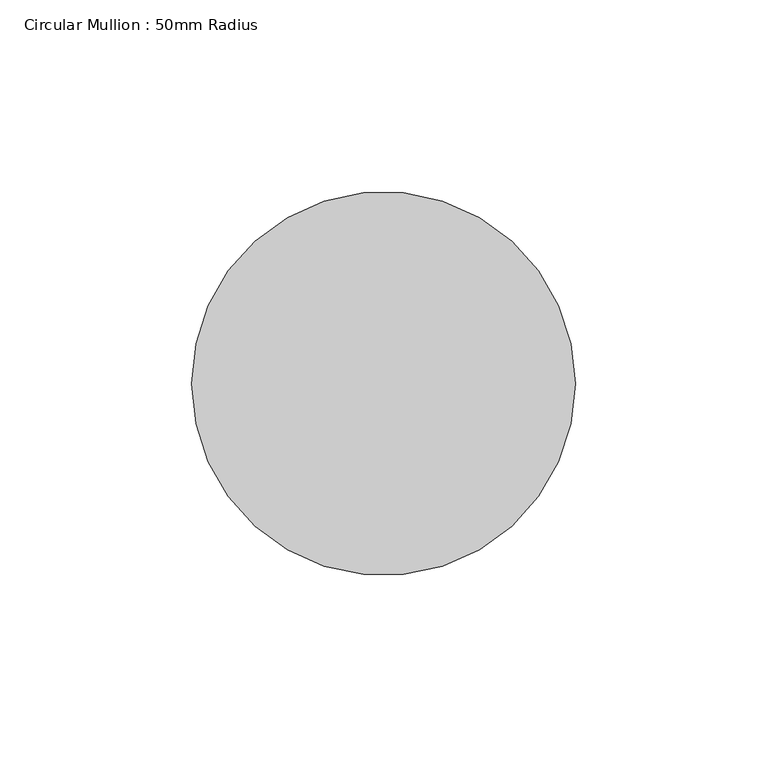
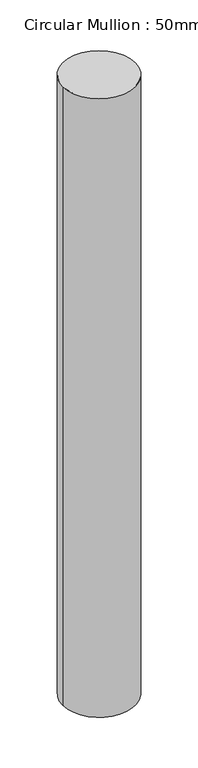
"""IFC4 building model written with IfcOpenShell, lengths in millimetres: member geometry, Circular Mullion : 50mm Radius."""

from ifc_helpers import new_model, si_unit, point, frame, origin, origin_2d, place, context, project, spatial, circle_curve, trimmed, segment, composite_curve, outline, extrude, source, transform, mapped, element, save


def circular_mullion_50mm_radius_88b615bb(model_context):
    return source(origin(), model_context, "Body", "SweptSolid", [
        extrude(outline(composite_curve([segment(trimmed(circle_curve(origin_2d(), 50.0), [point((50.0, 0.0))], [point((-50.0, 0.0))], False, "CARTESIAN"), True, "CONTINUOUS"), segment(trimmed(circle_curve(origin_2d(), 50.0), [point((-50.0, 0.0))], [point((50.0, 0.0))], False, "CARTESIAN"), True, "CONTINUOUS")], self_intersect=False)), frame((0.0, 0.0, -902.9152251), z_axis=(0.0, 0.0, 1.0), x_axis=(1.0, 0.0, 0.0)), (0.0, 0.0, 1.0), 902.9152251),
    ])


if __name__ == "__main__":
    model = new_model("IFC4")
    model_context = context("Model", 3, world=origin())
    ifc_project = project(units=[si_unit("LENGTHUNIT", "METRE", prefix="MILLI")], contexts=[model_context])
    site = spatial("IfcSite", under=ifc_project)
    building = spatial("IfcBuilding", under=site)
    placement = place(None, origin())
    circular_mullion_50mm_radius_shape = circular_mullion_50mm_radius_88b615bb(model_context)
    element("IfcMember", 1, ObjectType="Circular Mullion : 50mm Radius", at=placement, inside=building, context=model_context, shape_type="MappedRepresentation", body=[
        mapped(circular_mullion_50mm_radius_shape, transform((0.0, 0.0, 0.0), x_axis=(1.0, 0.0, 0.0), y_axis=(0.0, 1.0, 0.0), z_axis=(0.0, 0.0, 1.0))),
    ])
    save(model, "model.ifc")

# Revit data of these elements
# Type "Circular Mullion : 50mm Radius"
#   built-in parameter 1007350 = 0.164042 (stored number, unit not read)
# Element 1 (IfcMember, "Circular Mullion : 50mm Radius")
#   Materials on its faces: "Aluminium"
# Materials
#   "Aluminium": class "Metal", colour RGB 247 247 247, transparency 0, Description = "Aluminium 6061", Cost = 0
